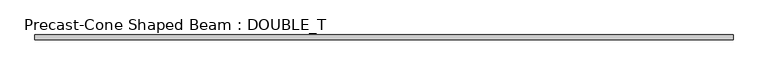
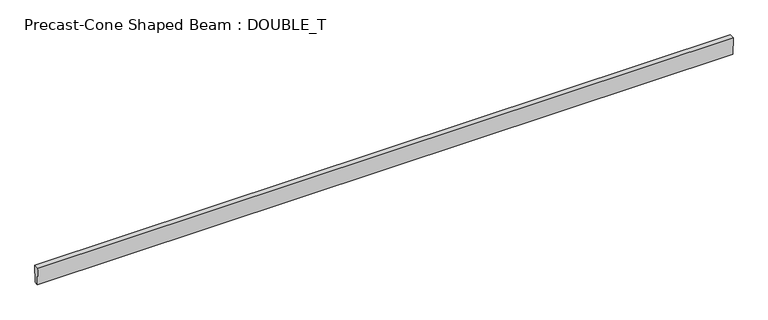
"""IFC4 building model written with IfcOpenShell, lengths in millimetres: beam geometry, Precast-Cone Shaped Beam : DOUBLE_T."""

from ifc_helpers import new_model, si_unit, frame, origin, place, context, project, spatial, polyline, outline, extrude, source, transform, mapped, element, save


def precast_cone_shaped_beam_double_t_b6a0bb25(model_context):
    return source(origin(), model_context, "Body", "SweptSolid", [
        extrude(outline(polyline([(-50.8, -228.6), (-63.5, 228.6), (63.5, 228.6), (50.8, -228.6), (-50.8, -228.6)])), frame((-8915.4, 0.0, 0.0), z_axis=(1.0, 0.0, 0.0), x_axis=(0.0, 1.0, 0.0)), (0.0, 0.0, 1.0), 17741.9),
    ])


if __name__ == "__main__":
    model = new_model("IFC4")
    model_context = context("Model", 3, world=origin())
    ifc_project = project(units=[si_unit("LENGTHUNIT", "METRE", prefix="MILLI")], contexts=[model_context])
    site = spatial("IfcSite", under=ifc_project)
    building = spatial("IfcBuilding", under=site)
    placement = place(None, origin())
    precast_cone_shaped_beam_double_t_shape = precast_cone_shaped_beam_double_t_b6a0bb25(model_context)
    element("IfcBeam", 1, ObjectType="Precast-Cone Shaped Beam : DOUBLE_T", at=placement, inside=building, context=model_context, shape_type="MappedRepresentation", body=[
        mapped(precast_cone_shaped_beam_double_t_shape, transform((0.0, 0.0, 0.0), x_axis=(1.0, 0.0, 0.0), y_axis=(0.0, 1.0, 0.0), z_axis=(0.0, 0.0, 1.0))),
    ])
    save(model, "model.ifc")

# Revit data of these elements
# Type "Precast-Cone Shaped Beam : DOUBLE_T"
#   Top Width = 0' - 5"
#   Tie Rod Weight [instance default] = 30
#   Tie Rod W [instance default] = 0.0660938 kip
#   Single Rebar Weight [instance default] = 50
#   Single Rebar W [instance default] = 0.110156 kip
#   Rebar Grids Weight [instance default] = 100
#   Rebar Grids W [instance default] = 0.220313 kip
#   Depth = 1' - 6"
#   Bottom Width = 0' - 4"
#   Length [instance default] = 5' - 0"
#   Structural Material [instance default] = Concrete, Precast
#   Assembly Code = ""
# Element 1 (IfcBeam, "Precast-Cone Shaped Beam : DOUBLE_T")
#   Length = 59' - 6"
#   Structural Material = Concrete - Precast Concrete - Normal Weight Concrete - 5 ksi
#   Materials on its faces: "Concrete - Precast Concrete - Normal Weight Concrete - 5 ksi"
# Materials
#   "Concrete, Precast": class "Concrete", colour RGB 198 187 187, transparency 0, Description = "Precast concrete", Cost = 0
#   "Concrete - Precast Concrete - Normal Weight Concrete - 5 ksi": class "Concrete", colour RGB 198 187 187, transparency 0, Cost = 0
